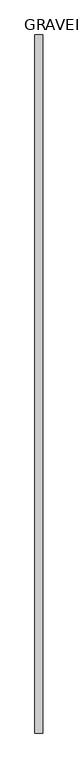
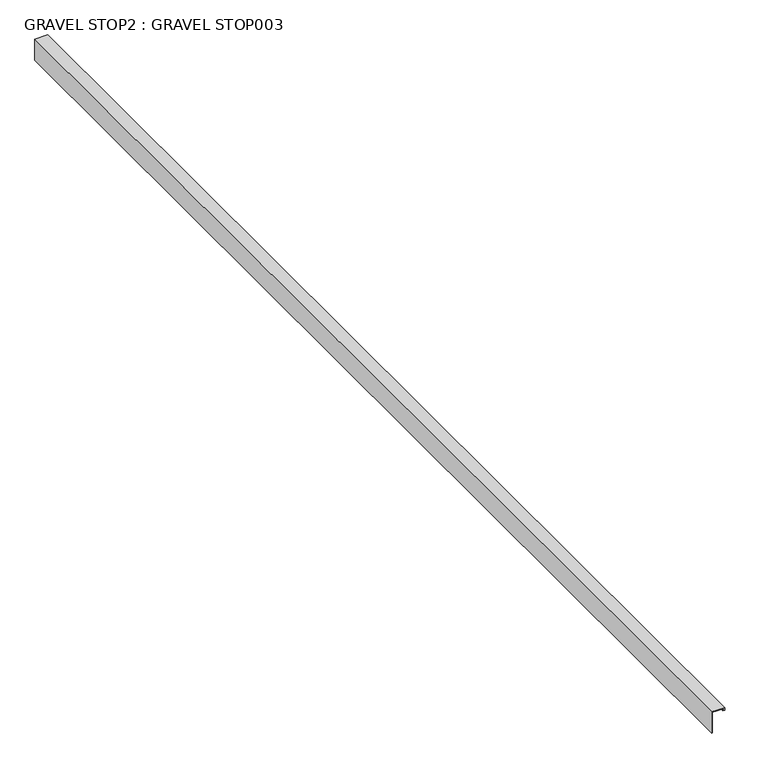
"""IFC4 building model written with IfcOpenShell, lengths in millimetres: proxy geometry, GRAVEL STOP2 : GRAVEL STOP003."""

import ifcopenshell
import ifcopenshell.guid

model = None  # the IFC model being written
_history = None  # IfcOwnerHistory: only IFC2X3 demands one
_inside = {}  # id of a spatial element -> (the spatial element, [elements in it])
_under = {}  # id of a project, library or spatial element -> (it, [spatial elements below it])
_declared = {}  # id of a project -> (the project, [libraries it declares])
_typed = {}  # id of a type object -> (the type object, [elements of that type])
_made_of = {}  # id of a material, layer set ... -> (it, [elements and type objects made of it])


def new_model(schema):
    """Start an empty IFC model of exactly this schema.

    Asked for "IFC4X3", IfcOpenShell would pick the latest addendum, in which some entities
    have other attributes; the version numbers below select the first issue.
    IFC2X3 requires an IfcOwnerHistory on every rooted entity: one is made here for all.
    """
    global model, _history
    if schema == "IFC4X3":
        model = ifcopenshell.file(schema_version=(4, 3, 0, 0))
    else:
        model = ifcopenshell.file(schema=schema)
    _inside.clear()
    _under.clear()
    _declared.clear()
    _typed.clear()
    _made_of.clear()
    _history = None
    if model.schema == "IFC2X3":
        org = make("IfcOrganization", Name="unknown")
        user = make(
            "IfcPersonAndOrganization",
            ThePerson=make("IfcPerson", FamilyName="unknown"),
            TheOrganization=org,
        )
        app = make(
            "IfcApplication",
            ApplicationDeveloper=org,
            Version="unknown",
            ApplicationFullName="unknown",
            ApplicationIdentifier="unknown",
        )
        _history = make(
            "IfcOwnerHistory",
            OwningUser=user,
            OwningApplication=app,
            ChangeAction="ADDED",
            CreationDate=0,
        )
    return model


def make(cls, **values):
    """One entity of the class cls with the attributes given. An attribute that is None is left unset."""
    return model.create_entity(
        cls, **{name: value for name, value in values.items() if value is not None}
    )


def rooted(cls, **values):
    """An entity with a GlobalId (a new one), such as an element, a storey or a relation."""
    return make(cls, GlobalId=ifcopenshell.guid.new(), OwnerHistory=_history, **values)


def si_unit(unit_type, name, prefix=None):
    """IfcSIUnit, for example si_unit("LENGTHUNIT", "METRE", prefix="MILLI")."""
    return make("IfcSIUnit", UnitType=unit_type, Prefix=prefix, Name=name)


def assignment(units):
    """IfcUnitAssignment: the units of a project."""
    return None if units is None else make("IfcUnitAssignment", Units=units)


def point(xyz):
    """IfcCartesianPoint."""
    return None if xyz is None else make("IfcCartesianPoint", Coordinates=xyz)


def direction(xyz):
    """IfcDirection."""
    return None if xyz is None else make("IfcDirection", DirectionRatios=xyz)


def frame(location, z_axis=None, x_axis=None):
    """IfcAxis2Placement3D, a coordinate frame: its origin and axes. An axis left out is left unset."""
    return make(
        "IfcAxis2Placement3D",
        Location=point(location),
        Axis=direction(z_axis),
        RefDirection=direction(x_axis),
    )


def origin():
    """The frame at (0, 0, 0) with its axes left unset."""
    return frame((0.0, 0.0, 0.0))


def place(relative_to, where):
    """IfcLocalPlacement: puts the frame where relative to a parent placement (None: the world)."""
    return make(
        "IfcLocalPlacement", PlacementRelTo=relative_to, RelativePlacement=where
    )


def context(
    kind, dimensions, precision=None, world=None, true_north=None, identifier=None
):
    """IfcGeometricRepresentationContext, for example the 3D "Model" context."""
    return make(
        "IfcGeometricRepresentationContext",
        ContextIdentifier=identifier,
        ContextType=kind,
        CoordinateSpaceDimension=dimensions,
        Precision=precision,
        WorldCoordinateSystem=world,
        TrueNorth=true_north,
    )


def project(units=None, contexts=None):
    """IfcProject with its units and contexts."""
    return rooted(
        "IfcProject",
        Name="project",
        RepresentationContexts=contexts,
        UnitsInContext=assignment(units),
    )


def spatial(cls, under=None, at=None, **own):
    """A site, building, storey or space (cls), placed at a placement, below another one or the project."""
    s = rooted(cls, ObjectPlacement=at, **own)
    if under is not None:
        _under.setdefault(under.id(), (under, []))[1].append(s)
    return s


def polyline(points):
    """IfcPolyline through the points."""
    return make("IfcPolyline", Points=[point(p) for p in points])


def outline(outer, holes=None, kind="AREA"):
    """IfcArbitraryClosedProfileDef: a profile drawn as a closed curve; with holes, ...WithVoids."""
    if holes is None:
        return make("IfcArbitraryClosedProfileDef", ProfileType=kind, OuterCurve=outer)
    return make(
        "IfcArbitraryProfileDefWithVoids",
        ProfileType=kind,
        OuterCurve=outer,
        InnerCurves=holes,
    )


def extrude(swept, where, along, depth):
    """IfcExtrudedAreaSolid: the profile swept, set in the frame where, extruded along a direction by depth."""
    return make(
        "IfcExtrudedAreaSolid",
        SweptArea=swept,
        Position=where,
        ExtrudedDirection=direction(along),
        Depth=depth,
    )


def shape(context_of_items, identifier, shape_type, items):
    """IfcShapeRepresentation: the items that make up one representation, for example the "Body"."""
    return make(
        "IfcShapeRepresentation",
        ContextOfItems=context_of_items,
        RepresentationIdentifier=identifier,
        RepresentationType=shape_type,
        Items=items,
    )


def source(mapping_origin, context_of_items, identifier, shape_type, items):
    """IfcRepresentationMap: a shape defined once, which mapped items show again and again."""
    return make(
        "IfcRepresentationMap",
        MappingOrigin=mapping_origin,
        MappedRepresentation=shape(context_of_items, identifier, shape_type, items),
    )


def transform(
    local_origin,
    x_axis=None,
    y_axis=None,
    z_axis=None,
    scale=None,
    scale2=None,
    scale3=None,
    uniform=True,
):
    """IfcCartesianTransformationOperator3D, or its non-uniform kind. x_axis, y_axis, z_axis: its Axis1, 2, 3."""
    if uniform:
        return make(
            "IfcCartesianTransformationOperator3D",
            Axis1=direction(x_axis),
            Axis2=direction(y_axis),
            LocalOrigin=point(local_origin),
            Scale=scale,
            Axis3=direction(z_axis),
        )
    return make(
        "IfcCartesianTransformationOperator3DnonUniform",
        Axis1=direction(x_axis),
        Axis2=direction(y_axis),
        LocalOrigin=point(local_origin),
        Scale=scale,
        Axis3=direction(z_axis),
        Scale2=scale2,
        Scale3=scale3,
    )


def mapped(mapping_source, mapping_target):
    """IfcMappedItem: shows the shape of a source again, moved by a transform."""
    return make(
        "IfcMappedItem", MappingSource=mapping_source, MappingTarget=mapping_target
    )


def made_of(thing, what):
    """Note that an element or type object is made of a material, layer set ...; save() writes the relation."""
    if what is not None:
        _made_of.setdefault(what.id(), (what, []))[1].append(thing)
    return thing


def element(
    cls,
    number,
    at=None,
    inside=None,
    cuts=None,
    type_object=None,
    material=None,
    context=None,
    identifier="Body",
    shape_type=None,
    held_by="IfcProductDefinitionShape",
    body=None,
    shapes=None,
    **own,
):
    """One element of the class cls, such as IfcWall. Its Tag is "e" and its number.

    at: its placement. inside: the storey or other place that contains it. cuts: it is an
    opening in that element (IfcRelVoidsElement). A single representation is given by context,
    identifier, shape_type and body (its items); several are given by shapes. held_by: the class
    of the entity that holds the representations. save() writes the other relations.
    """
    e = rooted(cls, Tag="e%d" % number, ObjectPlacement=at, **own)
    if body is not None:
        shapes = [shape(context, identifier, shape_type, body)]
    if shapes is not None:
        e.Representation = make(held_by, Representations=shapes)
    if inside is not None:
        _inside.setdefault(inside.id(), (inside, []))[1].append(e)
    if cuts is not None:
        rooted(
            "IfcRelVoidsElement", RelatingBuildingElement=cuts, RelatedOpeningElement=e
        )
    if type_object is not None:
        _typed.setdefault(type_object.id(), (type_object, []))[1].append(e)
    return made_of(e, material)


def aggregate(whole, parts):
    """IfcRelAggregates: a whole, such as a stair, and the parts it consists of."""
    return rooted("IfcRelAggregates", RelatingObject=whole, RelatedObjects=parts)


def save(model, path):
    """Write the relations noted so far, then the file.

    IfcRelAggregates (storeys below a building ...), IfcRelContainedInSpatialStructure (elements
    in a storey), IfcRelDefinesByType, IfcRelAssociatesMaterial and IfcRelDeclares: one each for
    every whole, place, type object, material and project.
    """
    for whole, parts in _under.values():
        aggregate(whole, parts)
    for where, things in _inside.values():
        rooted(
            "IfcRelContainedInSpatialStructure",
            RelatedElements=things,
            RelatingStructure=where,
        )
    for kind, things in _typed.values():
        rooted("IfcRelDefinesByType", RelatedObjects=things, RelatingType=kind)
    for what, things in _made_of.values():
        rooted("IfcRelAssociatesMaterial", RelatedObjects=things, RelatingMaterial=what)
    for by, libraries in _declared.values():
        rooted("IfcRelDeclares", RelatingContext=by, RelatedDefinitions=libraries)
    model.write(path)


def gravel_stop2_gravel_stop003_5ef83285(model_context):
    return source(origin(), model_context, "Body", "SweptSolid", [
        extrude(outline(polyline([(40234.4061757, -4378.3539248), (40234.4061757, -4358.6689248), (40232.1963757, -4358.6689248), (40232.1963757, -4360.4013812), (40230.9263757, -4360.4013812), (40230.9263757, -4357.3989248), (40235.6761757, -4357.3989248), (40235.6761757, -4379.6239248), (40197.5761757, -4379.6239248), (40197.5761757, -4378.3539248), (40234.4061757, -4378.3539248)])), frame((0.0, -1052.8906573, 0.0), z_axis=(0.0, 1.0, 0.0), x_axis=(0.0, 0.0, 1.0)), (0.0, 0.0, 1.0), 2000.25),
    ])


if __name__ == "__main__":
    model = new_model("IFC4")
    model_context = context("Model", 3, world=origin())
    ifc_project = project(units=[si_unit("LENGTHUNIT", "METRE", prefix="MILLI")], contexts=[model_context])
    site = spatial("IfcSite", under=ifc_project)
    building = spatial("IfcBuilding", under=site)
    placement = place(None, origin())
    gravel_stop2_gravel_stop003_shape = gravel_stop2_gravel_stop003_5ef83285(model_context)
    element("IfcBuildingElementProxy", 1, Name="GRAVEL STOP2 : GRAVEL STOP003", ObjectType="GRAVEL STOP2 : GRAVEL STOP003", at=placement, inside=building, context=model_context, shape_type="MappedRepresentation", body=[
        mapped(gravel_stop2_gravel_stop003_shape, transform((0.0, 0.0, 0.0), x_axis=(1.0, 0.0, 0.0), y_axis=(0.0, 1.0, 0.0), z_axis=(0.0, 0.0, 1.0))),
    ])
    save(model, "model.ifc")

# Revit data of these elements
# Type "GRAVEL STOP2 : GRAVEL STOP003"
#   NameOverride = "GRAVEL STOP003"
# Element 1 (IfcBuildingElementProxy, "GRAVEL STOP2 : GRAVEL STOP003")
#   Materials on its faces: "COPPER STUCCO J BEAD"
# Materials
#   "COPPER STUCCO J BEAD": class "Unassigned", colour RGB 251 232 155, transparency 0, Cost = 0
